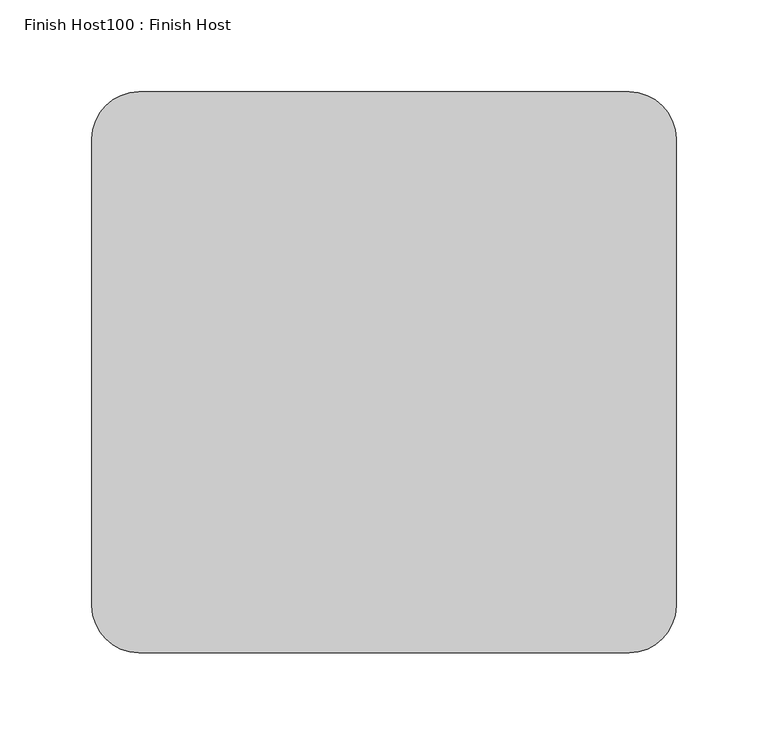
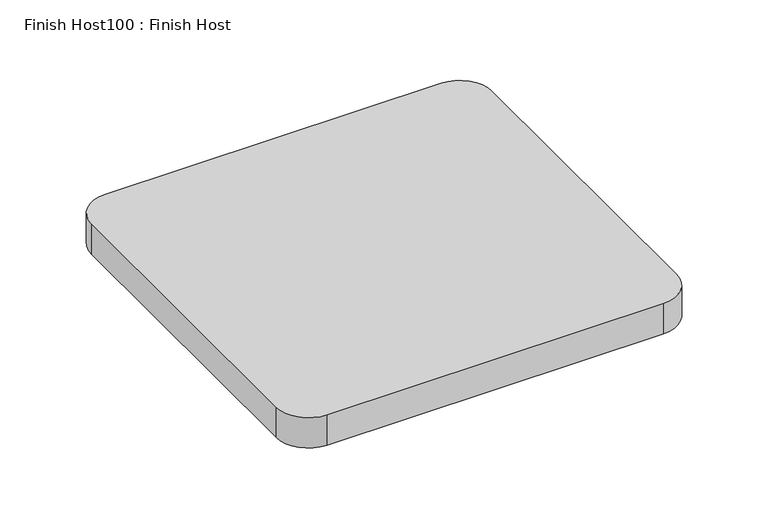
"""IFC4 building model written with IfcOpenShell, lengths in millimetres: proxy geometry, Finish Host100 : Finish Host."""

from ifc_helpers import new_model, si_unit, point, frame_2d, origin, origin_with_axes, place, context, project, spatial, polyline, circle_curve, trimmed, segment, composite_curve, outline, extrude, source, transform, mapped, element, save


def finish_host100_finish_host_594533e4(model_context):
    return source(origin(), model_context, "Body", "SweptSolid", [
        extrude(outline(composite_curve([segment(polyline([(-4689.5689884, -16767.3109369), (-4689.5689884, -16513.3109369)]), True, "CONTINUOUS"), segment(trimmed(circle_curve(frame_2d((-4664.1689884, -16513.3109369)), 25.4), [point((-4689.5689884, -16513.3109369))], [point((-4664.1689884, -16487.9109369))], False, "CARTESIAN"), True, "CONTINUOUS"), segment(polyline([(-4664.1689884, -16487.9109369), (-4397.4689884, -16487.9109369)]), True, "CONTINUOUS"), segment(trimmed(circle_curve(frame_2d((-4397.4689884, -16513.3109369)), 25.4), [point((-4397.4689884, -16487.9109369))], [point((-4372.0689884, -16513.3109369))], False, "CARTESIAN"), True, "CONTINUOUS"), segment(polyline([(-4372.0689884, -16513.3109369), (-4372.0689884, -16767.3109369)]), True, "CONTINUOUS"), segment(trimmed(circle_curve(frame_2d((-4397.4689884, -16767.3109369)), 25.4), [point((-4372.0689884, -16767.3109369))], [point((-4397.4689884, -16792.7109369))], False, "CARTESIAN"), True, "CONTINUOUS"), segment(polyline([(-4397.4689884, -16792.7109369), (-4664.1689884, -16792.7109369)]), True, "CONTINUOUS"), segment(trimmed(circle_curve(frame_2d((-4664.1689884, -16767.3109369)), 25.4), [point((-4664.1689884, -16792.7109369))], [point((-4689.5689884, -16767.3109369))], False, "CARTESIAN"), True, "CONTINUOUS")], self_intersect=False)), origin_with_axes(), (0.0, 0.0, 1.0), 25.4),
    ])


if __name__ == "__main__":
    model = new_model("IFC4")
    model_context = context("Model", 3, world=origin())
    ifc_project = project(units=[si_unit("LENGTHUNIT", "METRE", prefix="MILLI")], contexts=[model_context])
    site = spatial("IfcSite", under=ifc_project)
    building = spatial("IfcBuilding", under=site)
    placement = place(None, origin())
    finish_host100_finish_host_shape = finish_host100_finish_host_594533e4(model_context)
    element("IfcBuildingElementProxy", 1, Name="Finish Host100 : Finish Host", ObjectType="Finish Host100 : Finish Host", at=placement, inside=building, context=model_context, shape_type="MappedRepresentation", body=[
        mapped(finish_host100_finish_host_shape, transform((0.0, 0.0, 0.0), x_axis=(1.0, 0.0, 0.0), y_axis=(0.0, 1.0, 0.0), z_axis=(0.0, 0.0, 1.0))),
    ])
    save(model, "model.ifc")

# Revit data of these elements
# Type "Finish Host100 : Finish Host"
#   Countertop Material = Fabric - Teknion - P124 - Percept - Devotion
# Element 1 (IfcBuildingElementProxy, "Finish Host100 : Finish Host")
#   Materials on its faces: "Fabric - Teknion - P124 - Percept - Devotion"
# Materials
#   "Fabric - Teknion - P124 - Percept - Devotion": class "Generic", colour RGB 74 41 51, transparency 0, Model = "P124", Manufacturer = "Teknion Textiles", URL = "http://www.tekniontextiles.ca/", Description = "Devotion Percept", Cost = 0
